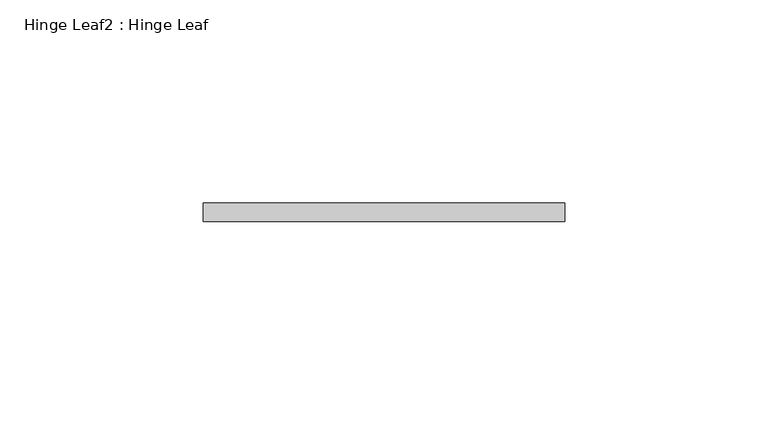
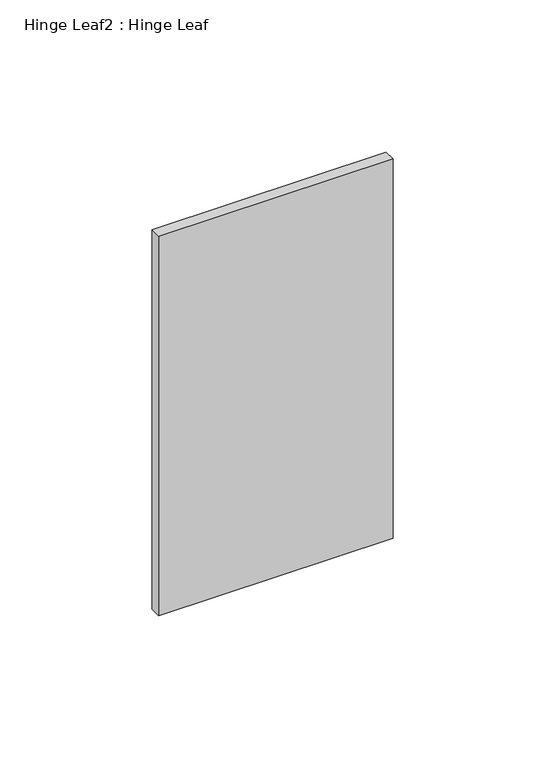
"""IFC4 building model written with IfcOpenShell, lengths in millimetres: proxy geometry, Hinge Leaf2 : Hinge Leaf."""

import ifcopenshell
import ifcopenshell.guid

model = None  # the IFC model being written
_history = None  # IfcOwnerHistory: only IFC2X3 demands one
_inside = {}  # id of a spatial element -> (the spatial element, [elements in it])
_under = {}  # id of a project, library or spatial element -> (it, [spatial elements below it])
_declared = {}  # id of a project -> (the project, [libraries it declares])
_typed = {}  # id of a type object -> (the type object, [elements of that type])
_made_of = {}  # id of a material, layer set ... -> (it, [elements and type objects made of it])


def new_model(schema):
    """Start an empty IFC model of exactly this schema.

    Asked for "IFC4X3", IfcOpenShell would pick the latest addendum, in which some entities
    have other attributes; the version numbers below select the first issue.
    IFC2X3 requires an IfcOwnerHistory on every rooted entity: one is made here for all.
    """
    global model, _history
    if schema == "IFC4X3":
        model = ifcopenshell.file(schema_version=(4, 3, 0, 0))
    else:
        model = ifcopenshell.file(schema=schema)
    _inside.clear()
    _under.clear()
    _declared.clear()
    _typed.clear()
    _made_of.clear()
    _history = None
    if model.schema == "IFC2X3":
        org = make("IfcOrganization", Name="unknown")
        user = make(
            "IfcPersonAndOrganization",
            ThePerson=make("IfcPerson", FamilyName="unknown"),
            TheOrganization=org,
        )
        app = make(
            "IfcApplication",
            ApplicationDeveloper=org,
            Version="unknown",
            ApplicationFullName="unknown",
            ApplicationIdentifier="unknown",
        )
        _history = make(
            "IfcOwnerHistory",
            OwningUser=user,
            OwningApplication=app,
            ChangeAction="ADDED",
            CreationDate=0,
        )
    return model


def make(cls, **values):
    """One entity of the class cls with the attributes given. An attribute that is None is left unset."""
    return model.create_entity(
        cls, **{name: value for name, value in values.items() if value is not None}
    )


def rooted(cls, **values):
    """An entity with a GlobalId (a new one), such as an element, a storey or a relation."""
    return make(cls, GlobalId=ifcopenshell.guid.new(), OwnerHistory=_history, **values)


def si_unit(unit_type, name, prefix=None):
    """IfcSIUnit, for example si_unit("LENGTHUNIT", "METRE", prefix="MILLI")."""
    return make("IfcSIUnit", UnitType=unit_type, Prefix=prefix, Name=name)


def assignment(units):
    """IfcUnitAssignment: the units of a project."""
    return None if units is None else make("IfcUnitAssignment", Units=units)


def point(xyz):
    """IfcCartesianPoint."""
    return None if xyz is None else make("IfcCartesianPoint", Coordinates=xyz)


def direction(xyz):
    """IfcDirection."""
    return None if xyz is None else make("IfcDirection", DirectionRatios=xyz)


def frame(location, z_axis=None, x_axis=None):
    """IfcAxis2Placement3D, a coordinate frame: its origin and axes. An axis left out is left unset."""
    return make(
        "IfcAxis2Placement3D",
        Location=point(location),
        Axis=direction(z_axis),
        RefDirection=direction(x_axis),
    )


def origin():
    """The frame at (0, 0, 0) with its axes left unset."""
    return frame((0.0, 0.0, 0.0))


def place(relative_to, where):
    """IfcLocalPlacement: puts the frame where relative to a parent placement (None: the world)."""
    return make(
        "IfcLocalPlacement", PlacementRelTo=relative_to, RelativePlacement=where
    )


def context(
    kind, dimensions, precision=None, world=None, true_north=None, identifier=None
):
    """IfcGeometricRepresentationContext, for example the 3D "Model" context."""
    return make(
        "IfcGeometricRepresentationContext",
        ContextIdentifier=identifier,
        ContextType=kind,
        CoordinateSpaceDimension=dimensions,
        Precision=precision,
        WorldCoordinateSystem=world,
        TrueNorth=true_north,
    )


def project(units=None, contexts=None):
    """IfcProject with its units and contexts."""
    return rooted(
        "IfcProject",
        Name="project",
        RepresentationContexts=contexts,
        UnitsInContext=assignment(units),
    )


def spatial(cls, under=None, at=None, **own):
    """A site, building, storey or space (cls), placed at a placement, below another one or the project."""
    s = rooted(cls, ObjectPlacement=at, **own)
    if under is not None:
        _under.setdefault(under.id(), (under, []))[1].append(s)
    return s


def polyline(points):
    """IfcPolyline through the points."""
    return make("IfcPolyline", Points=[point(p) for p in points])


def outline(outer, holes=None, kind="AREA"):
    """IfcArbitraryClosedProfileDef: a profile drawn as a closed curve; with holes, ...WithVoids."""
    if holes is None:
        return make("IfcArbitraryClosedProfileDef", ProfileType=kind, OuterCurve=outer)
    return make(
        "IfcArbitraryProfileDefWithVoids",
        ProfileType=kind,
        OuterCurve=outer,
        InnerCurves=holes,
    )


def extrude(swept, where, along, depth):
    """IfcExtrudedAreaSolid: the profile swept, set in the frame where, extruded along a direction by depth."""
    return make(
        "IfcExtrudedAreaSolid",
        SweptArea=swept,
        Position=where,
        ExtrudedDirection=direction(along),
        Depth=depth,
    )


def shape(context_of_items, identifier, shape_type, items):
    """IfcShapeRepresentation: the items that make up one representation, for example the "Body"."""
    return make(
        "IfcShapeRepresentation",
        ContextOfItems=context_of_items,
        RepresentationIdentifier=identifier,
        RepresentationType=shape_type,
        Items=items,
    )


def source(mapping_origin, context_of_items, identifier, shape_type, items):
    """IfcRepresentationMap: a shape defined once, which mapped items show again and again."""
    return make(
        "IfcRepresentationMap",
        MappingOrigin=mapping_origin,
        MappedRepresentation=shape(context_of_items, identifier, shape_type, items),
    )


def transform(
    local_origin,
    x_axis=None,
    y_axis=None,
    z_axis=None,
    scale=None,
    scale2=None,
    scale3=None,
    uniform=True,
):
    """IfcCartesianTransformationOperator3D, or its non-uniform kind. x_axis, y_axis, z_axis: its Axis1, 2, 3."""
    if uniform:
        return make(
            "IfcCartesianTransformationOperator3D",
            Axis1=direction(x_axis),
            Axis2=direction(y_axis),
            LocalOrigin=point(local_origin),
            Scale=scale,
            Axis3=direction(z_axis),
        )
    return make(
        "IfcCartesianTransformationOperator3DnonUniform",
        Axis1=direction(x_axis),
        Axis2=direction(y_axis),
        LocalOrigin=point(local_origin),
        Scale=scale,
        Axis3=direction(z_axis),
        Scale2=scale2,
        Scale3=scale3,
    )


def mapped(mapping_source, mapping_target):
    """IfcMappedItem: shows the shape of a source again, moved by a transform."""
    return make(
        "IfcMappedItem", MappingSource=mapping_source, MappingTarget=mapping_target
    )


def made_of(thing, what):
    """Note that an element or type object is made of a material, layer set ...; save() writes the relation."""
    if what is not None:
        _made_of.setdefault(what.id(), (what, []))[1].append(thing)
    return thing


def element(
    cls,
    number,
    at=None,
    inside=None,
    cuts=None,
    type_object=None,
    material=None,
    context=None,
    identifier="Body",
    shape_type=None,
    held_by="IfcProductDefinitionShape",
    body=None,
    shapes=None,
    **own,
):
    """One element of the class cls, such as IfcWall. Its Tag is "e" and its number.

    at: its placement. inside: the storey or other place that contains it. cuts: it is an
    opening in that element (IfcRelVoidsElement). A single representation is given by context,
    identifier, shape_type and body (its items); several are given by shapes. held_by: the class
    of the entity that holds the representations. save() writes the other relations.
    """
    e = rooted(cls, Tag="e%d" % number, ObjectPlacement=at, **own)
    if body is not None:
        shapes = [shape(context, identifier, shape_type, body)]
    if shapes is not None:
        e.Representation = make(held_by, Representations=shapes)
    if inside is not None:
        _inside.setdefault(inside.id(), (inside, []))[1].append(e)
    if cuts is not None:
        rooted(
            "IfcRelVoidsElement", RelatingBuildingElement=cuts, RelatedOpeningElement=e
        )
    if type_object is not None:
        _typed.setdefault(type_object.id(), (type_object, []))[1].append(e)
    return made_of(e, material)


def aggregate(whole, parts):
    """IfcRelAggregates: a whole, such as a stair, and the parts it consists of."""
    return rooted("IfcRelAggregates", RelatingObject=whole, RelatedObjects=parts)


def save(model, path):
    """Write the relations noted so far, then the file.

    IfcRelAggregates (storeys below a building ...), IfcRelContainedInSpatialStructure (elements
    in a storey), IfcRelDefinesByType, IfcRelAssociatesMaterial and IfcRelDeclares: one each for
    every whole, place, type object, material and project.
    """
    for whole, parts in _under.values():
        aggregate(whole, parts)
    for where, things in _inside.values():
        rooted(
            "IfcRelContainedInSpatialStructure",
            RelatedElements=things,
            RelatingStructure=where,
        )
    for kind, things in _typed.values():
        rooted("IfcRelDefinesByType", RelatedObjects=things, RelatingType=kind)
    for what, things in _made_of.values():
        rooted("IfcRelAssociatesMaterial", RelatedObjects=things, RelatingMaterial=what)
    for by, libraries in _declared.values():
        rooted("IfcRelDeclares", RelatingContext=by, RelatedDefinitions=libraries)
    model.write(path)


def hinge_leaf2_hinge_leaf_155bf624(model_context):
    return source(origin(), model_context, "Body", "SweptSolid", [
        extrude(outline(polyline([(587327.7934739, -531780.6943841), (587416.6934739, -531780.6943841), (587416.6934739, -531785.2663841), (587327.7934739, -531785.2663841), (587327.7934739, -531780.6943841)])), frame((0.0, 0.0, 311.15), z_axis=(0.0, 0.0, 1.0), x_axis=(1.0, 0.0, 0.0)), (0.0, 0.0, 1.0), 152.4),
    ])


if __name__ == "__main__":
    model = new_model("IFC4")
    model_context = context("Model", 3, world=origin())
    ifc_project = project(units=[si_unit("LENGTHUNIT", "METRE", prefix="MILLI")], contexts=[model_context])
    site = spatial("IfcSite", under=ifc_project)
    building = spatial("IfcBuilding", under=site)
    placement = place(None, origin())
    hinge_leaf2_hinge_leaf_shape = hinge_leaf2_hinge_leaf_155bf624(model_context)
    element("IfcBuildingElementProxy", 1, Name="Hinge Leaf2 : Hinge Leaf", ObjectType="Hinge Leaf2 : Hinge Leaf", at=placement, inside=building, context=model_context, shape_type="MappedRepresentation", body=[
        mapped(hinge_leaf2_hinge_leaf_shape, transform((0.0, 0.0, 0.0), x_axis=(1.0, 0.0, 0.0), y_axis=(0.0, 1.0, 0.0), z_axis=(0.0, 0.0, 1.0))),
    ])
    save(model, "model.ifc")

# Revit data of these elements
# Element 1 (IfcBuildingElementProxy, "Hinge Leaf2 : Hinge Leaf")
#   Materials on its faces: "6\"X6\" WELD-ON STL BUTT HINGE"
# Materials
#   "6\"X6\" WELD-ON STL BUTT HINGE": class "Metal", colour RGB 189 187 185, transparency 0, Description = "Carbon steel", Cost = 0
